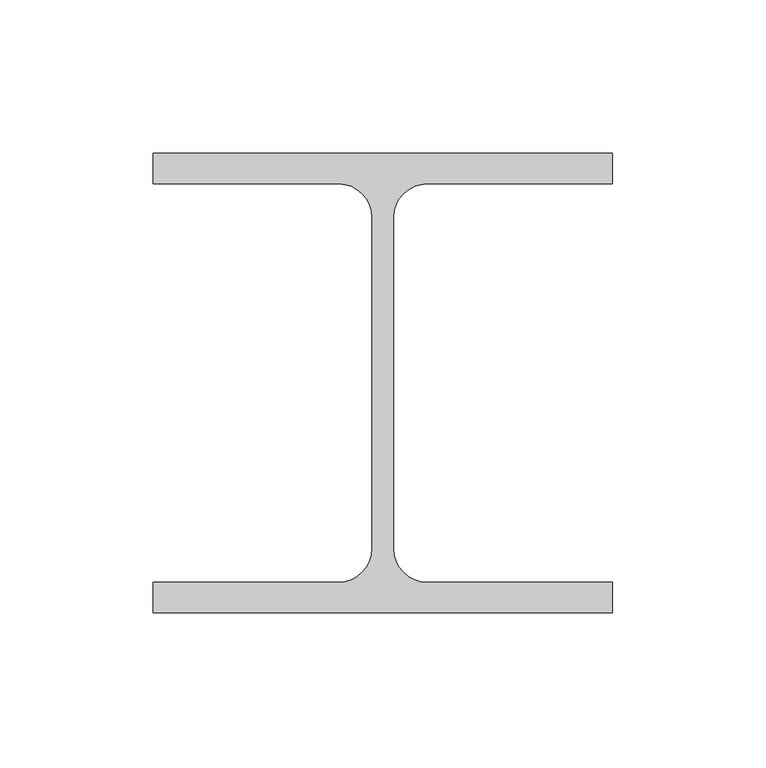
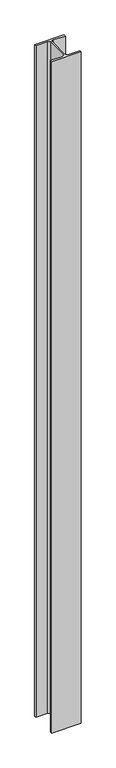
"""IFC4 building model written with IfcOpenShell, lengths in millimetres: column geometry, 0912_Steel Column_H_KSD3502 : H_SC_ASC_H-150x150x7x10."""

from ifc_helpers import new_model, si_unit, point, frame, frame_2d, origin, place, context, project, spatial, polyline, circle_curve, trimmed, segment, composite_curve, outline, extrude, source, transform, mapped, element, save


def column_0d026061(model_context):
    return source(origin(), model_context, "Body", "SweptSolid", [
        extrude(outline(composite_curve([segment(polyline([(75.0, 75.0), (75.0, 65.0), (14.5, 65.0)]), True, "CONTINUOUS"), segment(trimmed(circle_curve(frame_2d((14.5, 54.0)), 11.0), [point((14.5, 65.0))], [point((3.5, 54.0))], True, "CARTESIAN"), True, "CONTINUOUS"), segment(polyline([(3.5, 54.0), (3.5, -54.0)]), True, "CONTINUOUS"), segment(trimmed(circle_curve(frame_2d((14.5, -54.0)), 11.0), [point((3.5, -54.0))], [point((14.5, -65.0))], True, "CARTESIAN"), True, "CONTINUOUS"), segment(polyline([(14.5, -65.0), (75.0, -65.0), (75.0, -75.0), (-75.0, -75.0), (-75.0, -65.0), (-14.5, -65.0)]), True, "CONTINUOUS"), segment(trimmed(circle_curve(frame_2d((-14.5, -54.0)), 11.0), [point((-14.5, -65.0))], [point((-3.5, -54.0))], True, "CARTESIAN"), True, "CONTINUOUS"), segment(polyline([(-3.5, -54.0), (-3.5, 54.0)]), True, "CONTINUOUS"), segment(trimmed(circle_curve(frame_2d((-14.5, 54.0)), 11.0), [point((-3.5, 54.0))], [point((-14.5, 65.0))], True, "CARTESIAN"), True, "CONTINUOUS"), segment(polyline([(-14.5, 65.0), (-75.0, 65.0), (-75.0, 75.0), (75.0, 75.0)]), True, "CONTINUOUS")], self_intersect=False)), frame((0.0, 0.0, 8299.9720055), z_axis=(0.0, 0.0, 1.0), x_axis=(1.0, 0.0, 0.0)), (0.0, 0.0, 1.0), 3610.0),
    ])


if __name__ == "__main__":
    model = new_model("IFC4")
    model_context = context("Model", 3, world=origin())
    ifc_project = project(units=[si_unit("LENGTHUNIT", "METRE", prefix="MILLI")], contexts=[model_context])
    site = spatial("IfcSite", under=ifc_project)
    building = spatial("IfcBuilding", under=site)
    placement = place(None, origin())
    column_shape = column_0d026061(model_context)
    element("IfcColumn", 1, ObjectType="0912_Steel Column_H_KSD3502 : H_SC_ASC_H-150x150x7x10", at=placement, inside=building, context=model_context, shape_type="MappedRepresentation", body=[
        mapped(column_shape, transform((0.0, 0.0, 0.0), x_axis=(1.0, 0.0, 0.0), y_axis=(0.0, 1.0, 0.0), z_axis=(0.0, 0.0, 1.0))),
    ])
    save(model, "model.ifc")

# Revit data of these elements
# Type "0912_Steel Column_H_KSD3502 : H_SC_ASC_H-150x150x7x10"
#   H_WM Code_1 = "S01AA002-00001 | Main Steel Structure Fabrication Work | Shelter/Building | Medium Steel - Standard (90KG/M>Weight≥30KG/M) | Material: (   )"
#   H_WM Code_2 = "S03AA028-00001 | Main Steel Structure Erection Work | Shelter/Building | Medium Steel (90KG/M>Weight≥30KG/M) | Material: (   )"
#   H_WM Code_3 = "S01AA010-00001 | Main Steel Structure Fabrication Work | Shelter/Building | Steel Painting/Coating | for Non-Fireproofed Steel Surface, Surface Preparation, Primer, Second & Final Coat | Material: (   )"
#   H_Q'ty Cal Type Tag = "SC-Q2"
#   Width = 15.0 cm
#   Web Thickness = 0.7 cm
#   Web Fillet = 1.1 cm
#   Warping Constant = 27562.5 cm⁶
#   Torsional Moment of Inertia = 11.6007 cm⁴
#   Section Area = 40.14 cm²
#   Plastic Modulus weak axis = 115.0 cm³
#   Plastic Modulus strong axis = 246.0 cm³
#   Perimeter = 0.87 m²/m
#   Nominal Weight = 31.50 kgf/m
#   Moment of Inertia weak axis = 563.00 cm⁴
#   Moment of Inertia strong axis = 1640.00 cm⁴
#   Height = 15.0 cm
#   Flange Thickness = 1.0 cm
#   Elastic Modulus weak axis = 75.1 cm³
#   Elastic Modulus strong axis = 219.0 cm³
#   Centroid Vertical = 7.5 cm
#   Centroid Horizontal = 7.5 cm
#   Structural Material [instance default] = Steel, 45-345
#   Section Name Key = ""
#   Bolt Spacing = 0
#   Assembly Code = ""
# Element 1 (IfcColumn, "0912_Steel Column_H_KSD3502 : H_SC_ASC_H-150x150x7x10")
#   Structural Material = none
# Materials
#   "Steel, 45-345": class "Metal", colour RGB 189 187 185, transparency 0, Description = "Steel 345 MPa", Cost = 0
